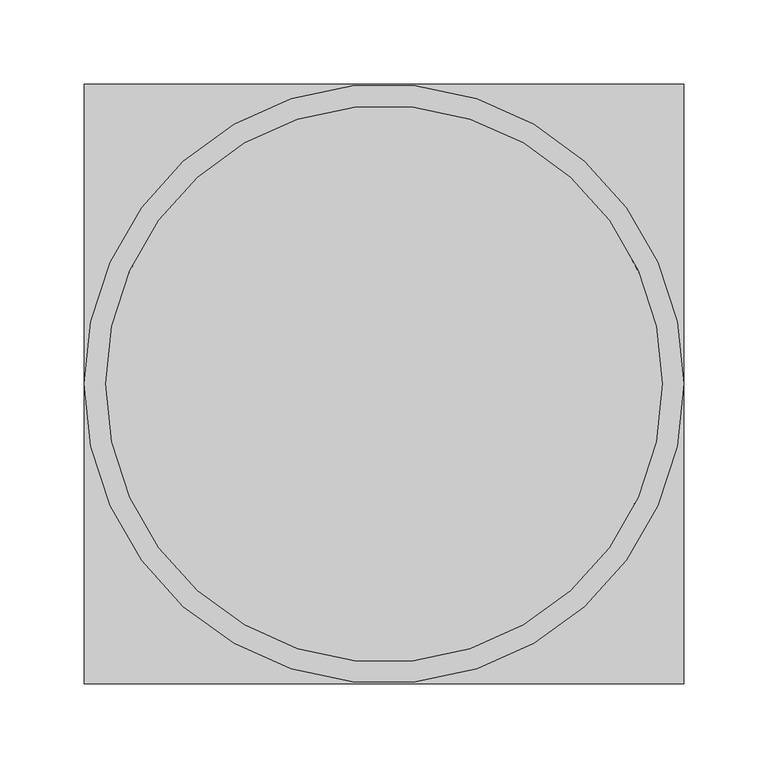
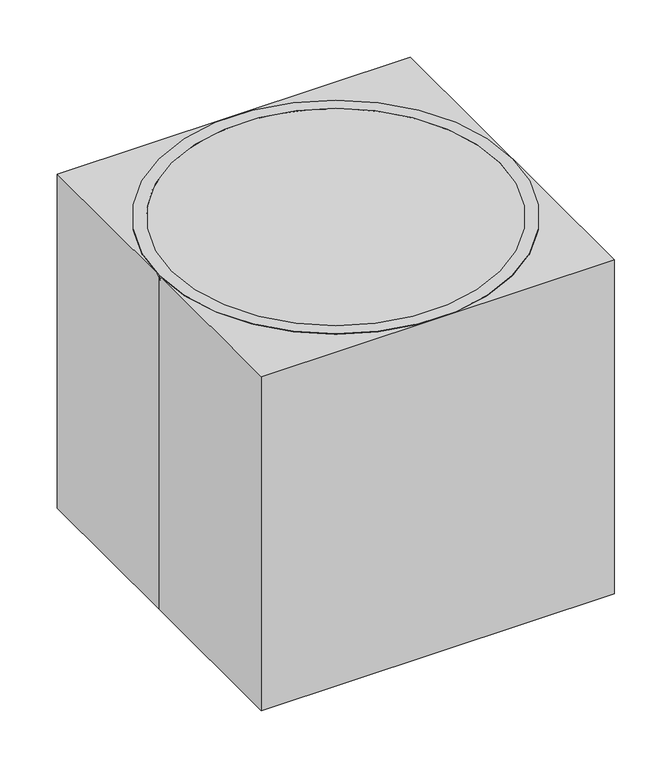
"""IFC4 building model written with IfcOpenShell, lengths in millimetres: proxy geometry, M8905 - Pail, Utility, CRS, Without Carriage : M8905 - Pail, Utility, CRS, Without Carriage."""

import ifcopenshell
import ifcopenshell.guid

model = None  # the IFC model being written
_history = None  # IfcOwnerHistory: only IFC2X3 demands one
_inside = {}  # id of a spatial element -> (the spatial element, [elements in it])
_under = {}  # id of a project, library or spatial element -> (it, [spatial elements below it])
_declared = {}  # id of a project -> (the project, [libraries it declares])
_typed = {}  # id of a type object -> (the type object, [elements of that type])
_made_of = {}  # id of a material, layer set ... -> (it, [elements and type objects made of it])


def new_model(schema):
    """Start an empty IFC model of exactly this schema.

    Asked for "IFC4X3", IfcOpenShell would pick the latest addendum, in which some entities
    have other attributes; the version numbers below select the first issue.
    IFC2X3 requires an IfcOwnerHistory on every rooted entity: one is made here for all.
    """
    global model, _history
    if schema == "IFC4X3":
        model = ifcopenshell.file(schema_version=(4, 3, 0, 0))
    else:
        model = ifcopenshell.file(schema=schema)
    _inside.clear()
    _under.clear()
    _declared.clear()
    _typed.clear()
    _made_of.clear()
    _history = None
    if model.schema == "IFC2X3":
        org = make("IfcOrganization", Name="unknown")
        user = make(
            "IfcPersonAndOrganization",
            ThePerson=make("IfcPerson", FamilyName="unknown"),
            TheOrganization=org,
        )
        app = make(
            "IfcApplication",
            ApplicationDeveloper=org,
            Version="unknown",
            ApplicationFullName="unknown",
            ApplicationIdentifier="unknown",
        )
        _history = make(
            "IfcOwnerHistory",
            OwningUser=user,
            OwningApplication=app,
            ChangeAction="ADDED",
            CreationDate=0,
        )
    return model


def make(cls, **values):
    """One entity of the class cls with the attributes given. An attribute that is None is left unset."""
    return model.create_entity(
        cls, **{name: value for name, value in values.items() if value is not None}
    )


def rooted(cls, **values):
    """An entity with a GlobalId (a new one), such as an element, a storey or a relation."""
    return make(cls, GlobalId=ifcopenshell.guid.new(), OwnerHistory=_history, **values)


def si_unit(unit_type, name, prefix=None):
    """IfcSIUnit, for example si_unit("LENGTHUNIT", "METRE", prefix="MILLI")."""
    return make("IfcSIUnit", UnitType=unit_type, Prefix=prefix, Name=name)


def assignment(units):
    """IfcUnitAssignment: the units of a project."""
    return None if units is None else make("IfcUnitAssignment", Units=units)


def point(xyz):
    """IfcCartesianPoint."""
    return None if xyz is None else make("IfcCartesianPoint", Coordinates=xyz)


def direction(xyz):
    """IfcDirection."""
    return None if xyz is None else make("IfcDirection", DirectionRatios=xyz)


def frame(location, z_axis=None, x_axis=None):
    """IfcAxis2Placement3D, a coordinate frame: its origin and axes. An axis left out is left unset."""
    return make(
        "IfcAxis2Placement3D",
        Location=point(location),
        Axis=direction(z_axis),
        RefDirection=direction(x_axis),
    )


def origin():
    """The frame at (0, 0, 0) with its axes left unset."""
    return frame((0.0, 0.0, 0.0))


def origin_with_axes():
    """The frame at (0, 0, 0) with the z axis (0, 0, 1) and the x axis (1, 0, 0) written out."""
    return frame((0.0, 0.0, 0.0), z_axis=(0.0, 0.0, 1.0), x_axis=(1.0, 0.0, 0.0))


def place(relative_to, where):
    """IfcLocalPlacement: puts the frame where relative to a parent placement (None: the world)."""
    return make(
        "IfcLocalPlacement", PlacementRelTo=relative_to, RelativePlacement=where
    )


def context(
    kind, dimensions, precision=None, world=None, true_north=None, identifier=None
):
    """IfcGeometricRepresentationContext, for example the 3D "Model" context."""
    return make(
        "IfcGeometricRepresentationContext",
        ContextIdentifier=identifier,
        ContextType=kind,
        CoordinateSpaceDimension=dimensions,
        Precision=precision,
        WorldCoordinateSystem=world,
        TrueNorth=true_north,
    )


def project(units=None, contexts=None):
    """IfcProject with its units and contexts."""
    return rooted(
        "IfcProject",
        Name="project",
        RepresentationContexts=contexts,
        UnitsInContext=assignment(units),
    )


def spatial(cls, under=None, at=None, **own):
    """A site, building, storey or space (cls), placed at a placement, below another one or the project."""
    s = rooted(cls, ObjectPlacement=at, **own)
    if under is not None:
        _under.setdefault(under.id(), (under, []))[1].append(s)
    return s


def polyline(points):
    """IfcPolyline through the points."""
    return make("IfcPolyline", Points=[point(p) for p in points])


def circle_curve(where, radius):
    """IfcCircle in the frame where."""
    return make("IfcCircle", Position=where, Radius=radius)


def outline(outer, holes=None, kind="AREA"):
    """IfcArbitraryClosedProfileDef: a profile drawn as a closed curve; with holes, ...WithVoids."""
    if holes is None:
        return make("IfcArbitraryClosedProfileDef", ProfileType=kind, OuterCurve=outer)
    return make(
        "IfcArbitraryProfileDefWithVoids",
        ProfileType=kind,
        OuterCurve=outer,
        InnerCurves=holes,
    )


def extrude(swept, where, along, depth):
    """IfcExtrudedAreaSolid: the profile swept, set in the frame where, extruded along a direction by depth."""
    return make(
        "IfcExtrudedAreaSolid",
        SweptArea=swept,
        Position=where,
        ExtrudedDirection=direction(along),
        Depth=depth,
    )


def shape(context_of_items, identifier, shape_type, items):
    """IfcShapeRepresentation: the items that make up one representation, for example the "Body"."""
    return make(
        "IfcShapeRepresentation",
        ContextOfItems=context_of_items,
        RepresentationIdentifier=identifier,
        RepresentationType=shape_type,
        Items=items,
    )


def source(mapping_origin, context_of_items, identifier, shape_type, items):
    """IfcRepresentationMap: a shape defined once, which mapped items show again and again."""
    return make(
        "IfcRepresentationMap",
        MappingOrigin=mapping_origin,
        MappedRepresentation=shape(context_of_items, identifier, shape_type, items),
    )


def transform(
    local_origin,
    x_axis=None,
    y_axis=None,
    z_axis=None,
    scale=None,
    scale2=None,
    scale3=None,
    uniform=True,
):
    """IfcCartesianTransformationOperator3D, or its non-uniform kind. x_axis, y_axis, z_axis: its Axis1, 2, 3."""
    if uniform:
        return make(
            "IfcCartesianTransformationOperator3D",
            Axis1=direction(x_axis),
            Axis2=direction(y_axis),
            LocalOrigin=point(local_origin),
            Scale=scale,
            Axis3=direction(z_axis),
        )
    return make(
        "IfcCartesianTransformationOperator3DnonUniform",
        Axis1=direction(x_axis),
        Axis2=direction(y_axis),
        LocalOrigin=point(local_origin),
        Scale=scale,
        Axis3=direction(z_axis),
        Scale2=scale2,
        Scale3=scale3,
    )


def mapped(mapping_source, mapping_target):
    """IfcMappedItem: shows the shape of a source again, moved by a transform."""
    return make(
        "IfcMappedItem", MappingSource=mapping_source, MappingTarget=mapping_target
    )


def made_of(thing, what):
    """Note that an element or type object is made of a material, layer set ...; save() writes the relation."""
    if what is not None:
        _made_of.setdefault(what.id(), (what, []))[1].append(thing)
    return thing


def element(
    cls,
    number,
    at=None,
    inside=None,
    cuts=None,
    type_object=None,
    material=None,
    context=None,
    identifier="Body",
    shape_type=None,
    held_by="IfcProductDefinitionShape",
    body=None,
    shapes=None,
    **own,
):
    """One element of the class cls, such as IfcWall. Its Tag is "e" and its number.

    at: its placement. inside: the storey or other place that contains it. cuts: it is an
    opening in that element (IfcRelVoidsElement). A single representation is given by context,
    identifier, shape_type and body (its items); several are given by shapes. held_by: the class
    of the entity that holds the representations. save() writes the other relations.
    """
    e = rooted(cls, Tag="e%d" % number, ObjectPlacement=at, **own)
    if body is not None:
        shapes = [shape(context, identifier, shape_type, body)]
    if shapes is not None:
        e.Representation = make(held_by, Representations=shapes)
    if inside is not None:
        _inside.setdefault(inside.id(), (inside, []))[1].append(e)
    if cuts is not None:
        rooted(
            "IfcRelVoidsElement", RelatingBuildingElement=cuts, RelatedOpeningElement=e
        )
    if type_object is not None:
        _typed.setdefault(type_object.id(), (type_object, []))[1].append(e)
    return made_of(e, material)


def aggregate(whole, parts):
    """IfcRelAggregates: a whole, such as a stair, and the parts it consists of."""
    return rooted("IfcRelAggregates", RelatingObject=whole, RelatedObjects=parts)


def save(model, path):
    """Write the relations noted so far, then the file.

    IfcRelAggregates (storeys below a building ...), IfcRelContainedInSpatialStructure (elements
    in a storey), IfcRelDefinesByType, IfcRelAssociatesMaterial and IfcRelDeclares: one each for
    every whole, place, type object, material and project.
    """
    for whole, parts in _under.values():
        aggregate(whole, parts)
    for where, things in _inside.values():
        rooted(
            "IfcRelContainedInSpatialStructure",
            RelatedElements=things,
            RelatingStructure=where,
        )
    for kind, things in _typed.values():
        rooted("IfcRelDefinesByType", RelatedObjects=things, RelatingType=kind)
    for what, things in _made_of.values():
        rooted("IfcRelAssociatesMaterial", RelatedObjects=things, RelatingMaterial=what)
    for by, libraries in _declared.values():
        rooted("IfcRelDeclares", RelatingContext=by, RelatedDefinitions=libraries)
    model.write(path)


def plane_surface(at):
    """IfcPlane: the flat surface through the origin of the frame at, square to its z axis."""
    return make("IfcPlane", Position=at)


def revolved_surface(curve, axis_point, axis_direction):
    """IfcSurfaceOfRevolution: the curve turned about the line through axis_point along axis_direction."""
    return make(
        "IfcSurfaceOfRevolution",
        SweptCurve=make("IfcArbitraryOpenProfileDef", ProfileType="CURVE", Curve=curve),
        AxisPosition=make("IfcAxis1Placement", Location=point(axis_point), Axis=direction(axis_direction)),
    )


def advanced_brep(points, edges, surfaces, faces):
    """IfcAdvancedBrep: a solid bounded by faces that lie on surfaces and meet in shared edges.

    An edge is (start, end): straight between two places in points (the first is 0);
    or (start, end, curve); or (start, end, curve, False) where it runs against its curve.
    A face is (place in surfaces, loops), or (place, loops, False) where it looks against
    its surface's normal. A loop lists edges by number (the first is 1), with a minus sign
    where the edge is run from its end to its start. The first loop is the outer one.
    """
    corners = [point(p) for p in points]
    vertices = [make("IfcVertexPoint", VertexGeometry=c) for c in corners]
    made = []
    for start, end, *more in edges:
        made.append(
            make(
                "IfcEdgeCurve",
                EdgeStart=vertices[start],
                EdgeEnd=vertices[end],
                EdgeGeometry=more[0] if more else make("IfcPolyline", Points=[corners[start], corners[end]]),
                SameSense=more[1] if len(more) > 1 else True,
            )
        )
    hull = []
    for where, loops, *sense in faces:
        bounds = []
        for j, loop in enumerate(loops):
            ring = [make("IfcOrientedEdge", EdgeElement=made[abs(k) - 1], Orientation=k > 0) for k in loop]
            bounds.append(
                make(
                    "IfcFaceOuterBound" if j == 0 else "IfcFaceBound",
                    Bound=make("IfcEdgeLoop", EdgeList=ring),
                    Orientation=True,
                )
            )
        hull.append(make("IfcAdvancedFace", Bounds=bounds, FaceSurface=surfaces[where], SameSense=sense[0] if sense else True))
    return make("IfcAdvancedBrep", Outer=make("IfcClosedShell", CfsFaces=hull))


def specialty_equipment_3ea2efa6(model_context):
    return source(origin(), model_context, "Body", "SolidModel", [
        advanced_brep(
        [(-127.0, 0.0, 0.0), (127.0, 0.0, 0.0), (-177.8, 0.0, 355.6), (177.8, 0.0, 355.6), (-165.1, 0.0, 355.6), (165.1, 0.0, 355.6), (114.3, 0.0, 19.5959229), (-114.3, 0.0, 19.5959229)],
        [
            (0, 1, circle_curve(frame((0.0, 0.0, 0.0), z_axis=(0.0, 0.0, -1.0), x_axis=(1.0, 0.0, 0.0)), 127.0)),
            (1, 0, circle_curve(frame((0.0, 0.0, 0.0), z_axis=(0.0, 0.0, -1.0), x_axis=(-1.0, 0.0, 0.0)), 127.0)),
            (2, 3, circle_curve(frame((0.0, 0.0, 355.6), z_axis=(0.0, 0.0, 1.0), x_axis=(-1.0, 0.0, 0.0)), 177.8)),
            (3, 2, circle_curve(frame((0.0, 0.0, 355.6), z_axis=(0.0, 0.0, 1.0), x_axis=(1.0, 0.0, 0.0)), 177.8)),
            (4, 5, circle_curve(frame((0.0, 0.0, 355.6), z_axis=(0.0, 0.0, -1.0), x_axis=(1.0, 0.0, 0.0)), 165.1)),
            (5, 4, circle_curve(frame((0.0, 0.0, 355.6), z_axis=(0.0, 0.0, -1.0), x_axis=(-1.0, 0.0, 0.0)), 165.1)),
            (0, 2),
            (3, 1),
            (6, 7, circle_curve(frame((0.0, 0.0, 19.5959229), z_axis=(0.0, 0.0, 1.0), x_axis=(1.0, 0.0, 0.0)), 114.3)),
            (7, 6, circle_curve(frame((0.0, 0.0, 19.5959229), z_axis=(0.0, 0.0, 1.0), x_axis=(-1.0, 0.0, 0.0)), 114.3)),
            (7, 4),
            (5, 6),
        ],
        [
            plane_surface(frame((0.0, 0.0, 0.0), z_axis=(0.0, 0.0, -1.0), x_axis=(0.0, 1.0, 0.0))),
            plane_surface(frame((0.0, 0.0, 355.6), z_axis=(0.0, 0.0, 1.0), x_axis=(0.0, 1.0, 0.0))),
            revolved_surface(polyline([(-127.00000000000001, 0.0, 0.0), (-177.8, 0.0, 355.5999999999999)]), (0.0, 0.0, -889.0), (0.0, 0.0, 1.0)),
            revolved_surface(polyline([(127.00000000000001, 0.0, 0.0), (177.8, 0.0, 355.5999999999999)]), (0.0, 0.0, -889.0), (0.0, 0.0, 1.0)),
            plane_surface(frame((0.0, 0.0, 19.5959229), z_axis=(0.0, 0.0, 1.0), x_axis=(0.0, 1.0, 0.0))),
            revolved_surface(polyline([(-165.1, 0.0, 355.60000000000014), (-114.299999996511, 0.0, 19.595922900000005)]), (0.0, 0.0, -736.4132505), (0.0, 0.0, 1.0)),
            revolved_surface(polyline([(165.1, 0.0, 355.60000000000014), (114.299999996511, 0.0, 19.595922900000005)]), (0.0, 0.0, -736.4132505), (0.0, 0.0, 1.0)),
        ],
        [
            (0, [[1, 2]]),
            (1, [[3, 4], [5, 6]]),
            (2, [[7, -4, 8, -1]]),
            (3, [[-8, -3, -7, -2]]),
            (4, [[9, 10]]),
            (5, [[11, -6, 12, -10]]),
            (6, [[-12, -5, -11, -9]]),
        ],
    ),
        extrude(outline(polyline([(-177.8, -177.8), (-177.8, 0.0), (-177.8, 177.8), (177.8, 177.8), (177.8, -177.8), (-177.8, -177.8)])), origin_with_axes(), (0.0, 0.0, 1.0), 355.6),
    ])


if __name__ == "__main__":
    model = new_model("IFC4")
    model_context = context("Model", 3, world=origin())
    ifc_project = project(units=[si_unit("LENGTHUNIT", "METRE", prefix="MILLI")], contexts=[model_context])
    site = spatial("IfcSite", under=ifc_project)
    building = spatial("IfcBuilding", under=site)
    placement = place(None, origin())
    specialty_equipment_shape = specialty_equipment_3ea2efa6(model_context)
    element("IfcBuildingElementProxy", 1, Name="M8905 - Pail, Utility, CRS, Without Carriage : M8905 - Pail, Utility, CRS, Without Carriage", ObjectType="M8905 - Pail, Utility, CRS, Without Carriage : M8905 - Pail, Utility, CRS, Without Carriage", at=placement, inside=building, context=model_context, shape_type="MappedRepresentation", body=[
        mapped(specialty_equipment_shape, transform((0.0, 0.0, 0.0), x_axis=(1.0, 0.0, 0.0), y_axis=(0.0, 1.0, 0.0), z_axis=(0.0, 0.0, 1.0))),
    ])
    save(model, "model.ifc")

# Revit data of these elements
# Type "M8905 - Pail, Utility, CRS, Without Carriage : M8905 - Pail, Utility, CRS, Without Carriage"
#   Watts2 = "0"
#   Watts1 = "0"
#   Unit_Issue = "EA"
#   UTIL_6_Misc = "-"
#   UTIL_5_NonMedGas = "-"
#   UTIL_4_MiscGas = "-"
#   UTIL_3_MedGas = "-"
#   UTIL_2_Elec = "-"
#   UTIL_1_WaterDrain = "-"
#   Nomenclature = "Pail, Utility, CRS, Without Carriage"
#   NSN = "6530"
#   Location [instance default] = ""
#   JSN = "M8905"
#   Fund_Source_VA = "-"
#   Fund_Source_Navy = "-"
#   Fund_Source_Army = "-"
#   Fund_Source_AF = "-"
#   ELEC_Volts2 = "0"
#   ELEC_Volts1 = "0"
#   ELEC_Phase2 = "0"
#   ELEC_Phase1 = "0"
#   ELEC_HertzSwitch = "0"
#   ELEC_HertzDependent = "0"
#   ELEC_Hertz = "0"
#   ELEC_Amps2 = "0"
#   ELEC_Amps1 = "0"
#   DetailDescription = "Utility pail (kick bucket). Shall be a stainless steel 12 quart bucket for use in surgical operating rooms."
#   CAT_VA = "C"
#   CAT_Navy = "C"
#   CAT_IHS = "-"
#   CAT_Army = "C"
#   CAT_AF = "C"
#   BTUperhour = "0"
#   Weight_IP = 12
#   DIM_Width_IP = 1' - 2"
#   DIM_Height_IP = 1' - 2"
#   DIM_Depth_IP = 1' - 2"
#   finish [instance default] = none
# Element 1 (IfcBuildingElementProxy, "M8905 - Pail, Utility, CRS, Without Carriage : M8905 - Pail, Utility, CRS, Without Carriage")
#   Location = "ORCS1"
#   Materials on its faces: "EquipSpace"
# Materials
#   "EquipSpace": class "Unassigned", colour RGB 221 217 195, transparency 0.5
